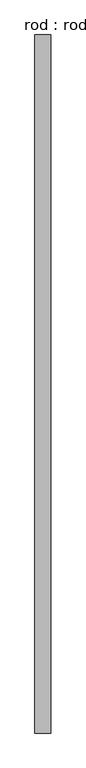
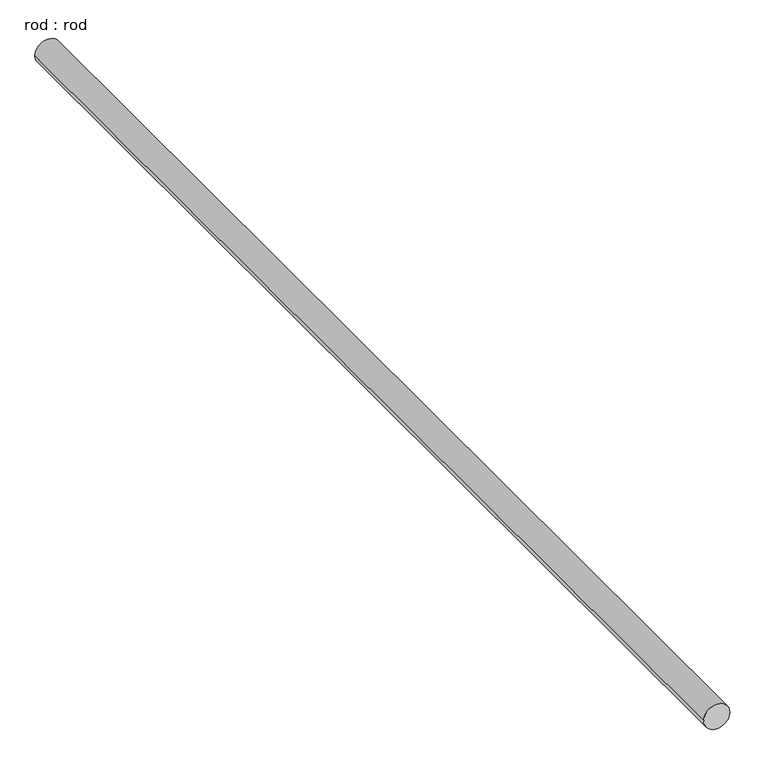
"""IFC4 building model written with IfcOpenShell, lengths in millimetres: proxy geometry, rod : rod."""

from ifc_helpers import new_model, si_unit, point, frame, frame_2d, origin, place, context, project, spatial, circle_curve, trimmed, segment, composite_curve, outline, extrude, source, transform, mapped, element, save


def rod_rod_a016ab76(model_context):
    return source(origin(), model_context, "Body", "SweptSolid", [
        extrude(outline(composite_curve([segment(trimmed(circle_curve(frame_2d((0.0108462, 0.0)), 200.0), [point((0.0108462, 200.0))], [point((0.0108462, -200.0))], False, "CARTESIAN"), True, "CONTINUOUS"), segment(trimmed(circle_curve(frame_2d((0.0108462, 0.0)), 200.0), [point((0.0108462, -200.0))], [point((0.0108462, 200.0))], False, "CARTESIAN"), True, "CONTINUOUS")], self_intersect=False)), frame((0.0, -4800.1285275, 0.0), z_axis=(0.0, 1.0, 0.0), x_axis=(0.0, 0.0, 1.0)), (0.0, 0.0, 1.0), 17785.7142857),
    ])


if __name__ == "__main__":
    model = new_model("IFC4")
    model_context = context("Model", 3, world=origin())
    ifc_project = project(units=[si_unit("LENGTHUNIT", "METRE", prefix="MILLI")], contexts=[model_context])
    site = spatial("IfcSite", under=ifc_project)
    building = spatial("IfcBuilding", under=site)
    placement = place(None, origin())
    rod_rod_shape = rod_rod_a016ab76(model_context)
    element("IfcBuildingElementProxy", 1, Name="rod : rod", ObjectType="rod : rod", at=placement, inside=building, context=model_context, shape_type="MappedRepresentation", body=[
        mapped(rod_rod_shape, transform((0.0, 0.0, 0.0), x_axis=(1.0, 0.0, 0.0), y_axis=(0.0, 1.0, 0.0), z_axis=(0.0, 0.0, 1.0))),
    ])
    save(model, "model.ifc")

# Revit data of these elements
# Type "rod : rod"
#   Default Elevation = 0
